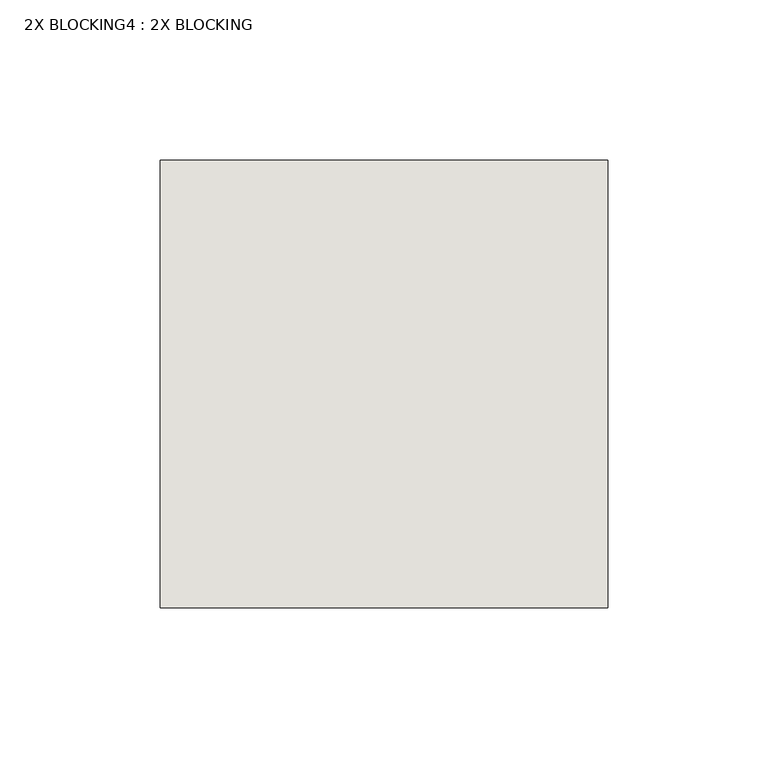
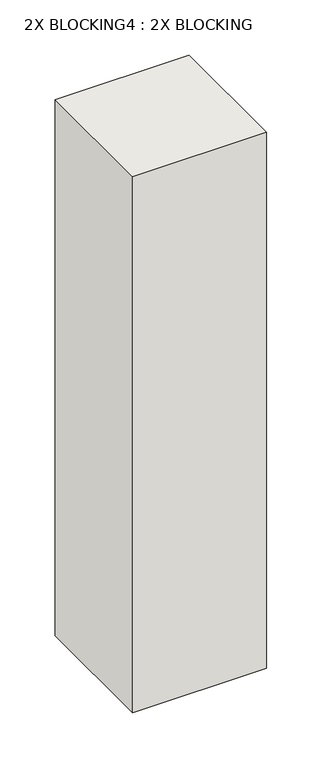
"""IFC4 building model written with IfcOpenShell, lengths in millimetres: wall geometry, 2X BLOCKING4 : 2X BLOCKING."""

from ifc_helpers import new_model, si_unit, frame, origin, place, context, project, spatial, polyline, outline, extrude, source, transform, mapped, element, save


def wall_2x_blocking4_2x_blocking_535ecf8f(model_context):
    return source(origin(), model_context, "Body", "SweptSolid", [
        extrude(outline(polyline([(23279.8870052, -1256.0384634), (23140.1870052, -1256.0384634), (23140.1870052, -1116.3384634), (23279.8870052, -1116.3384634), (23279.8870052, -1256.0384634)])), frame((0.0, 0.0, 4456.2028105), z_axis=(0.0, 0.0, 1.0), x_axis=(1.0, 0.0, 0.0)), (0.0, 0.0, 1.0), 590.55),
    ])


if __name__ == "__main__":
    model = new_model("IFC4")
    model_context = context("Model", 3, world=origin())
    ifc_project = project(units=[si_unit("LENGTHUNIT", "METRE", prefix="MILLI")], contexts=[model_context])
    site = spatial("IfcSite", under=ifc_project)
    building = spatial("IfcBuilding", under=site)
    placement = place(None, origin())
    wall_2x_blocking4_2x_blocking_shape = wall_2x_blocking4_2x_blocking_535ecf8f(model_context)
    element("IfcWall", 1, ObjectType="2X BLOCKING4 : 2X BLOCKING", at=placement, inside=building, context=model_context, shape_type="MappedRepresentation", body=[
        mapped(wall_2x_blocking4_2x_blocking_shape, transform((0.0, 0.0, 0.0), x_axis=(1.0, 0.0, 0.0), y_axis=(0.0, 1.0, 0.0), z_axis=(0.0, 0.0, 1.0))),
    ])
    save(model, "model.ifc")

# Revit data of these elements
# Type "2X BLOCKING4 : 2X BLOCKING"
#   Structural Material = 2 X BLOCKING
# Element 1 (IfcWall, "2X BLOCKING4 : 2X BLOCKING")
#   Materials on its faces: "2X6 STUD BEYOND"
# Materials
#   "2 X BLOCKING": class "Wood", colour RGB 234 198 147, transparency 0, Description = "Pinus Echinata", Cost = 0
#   "2X6 STUD BEYOND": class "Wood", colour RGB 234 198 147, transparency 0, Description = "Pinus Echinata", Cost = 0
